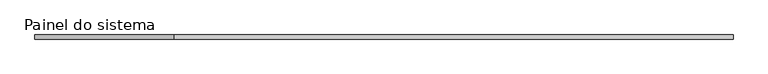
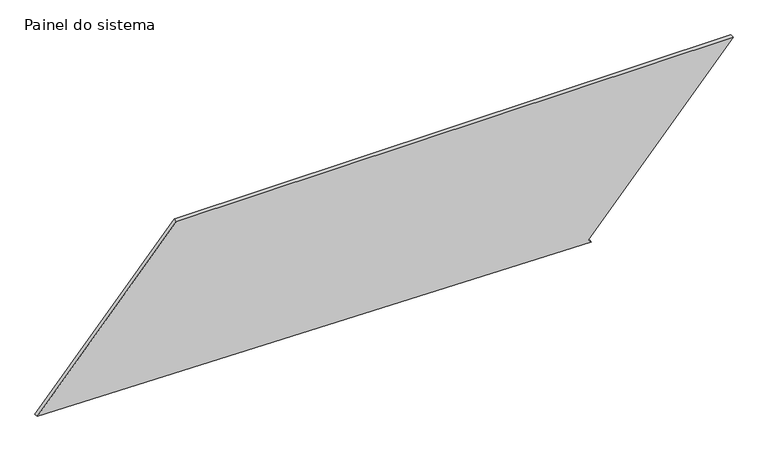
"""IFC4 building model written with IfcOpenShell, lengths in millimetres: plate geometry, Painel do sistema : Envidraçado."""

from ifc_helpers import new_model, si_unit, frame, origin, place, context, project, spatial, polyline, outline, extrude, source, transform, mapped, element, save


def painel_do_sistema_b5e2aceb(model_context):
    return source(origin(), model_context, "Body", "SweptSolid", [
        extrude(outline(polyline([(0.0, 1258.1615747), (16.5356636, 1239.4113259), (1018.231214, 2122.7969769), (1018.231214, -1273.9965643), (55.752827, -2122.7969769), (0.0, 1258.1615747)])), frame((0.0, 24.5, 0.0), z_axis=(0.0, 1.0, 0.0), x_axis=(0.0, 0.0, 1.0)), (0.0, 0.0, 1.0), 25.0),
    ])


if __name__ == "__main__":
    model = new_model("IFC4")
    model_context = context("Model", 3, world=origin())
    ifc_project = project(units=[si_unit("LENGTHUNIT", "METRE", prefix="MILLI")], contexts=[model_context])
    site = spatial("IfcSite", under=ifc_project)
    building = spatial("IfcBuilding", under=site)
    placement = place(None, origin())
    painel_do_sistema_shape = painel_do_sistema_b5e2aceb(model_context)
    element("IfcPlate", 1, ObjectType="Painel do sistema : Envidraçado", at=placement, inside=building, context=model_context, shape_type="MappedRepresentation", body=[
        mapped(painel_do_sistema_shape, transform((0.0, 0.0, 0.0), x_axis=(1.0, 0.0, 0.0), y_axis=(0.0, 1.0, 0.0), z_axis=(0.0, 0.0, 1.0))),
    ])
    save(model, "model.ifc")

# Revit data of these elements
# Type "Painel do sistema : Envidraçado"
#   Construction Type Id = "GSP4R"
#   Analytic Construction = "Vidraça única Pilkington 1/8 pol"
#   Visual Light Transmittance = 0.9
#   Solar Heat Gain Coefficient = 0.86
#   Heat Transfer Coefficient (U) = 6.7069 W/(m²·K)
# Element 1 (IfcPlate, "Painel do sistema : Envidraçado")
#   Materials on its faces: "Vidro"
# Materials
#   "Vidro": class "Vidro", colour RGB 0 128 192, transparency 0.9, Description = "Vidro de sílica", Cost = 0
